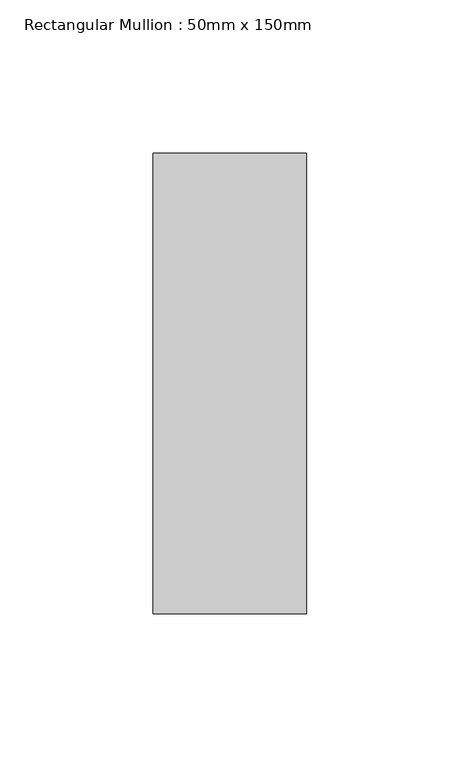
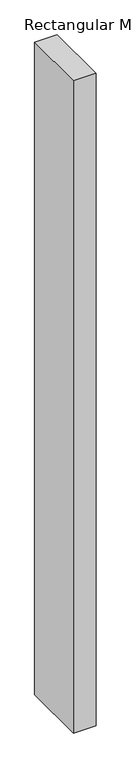
"""IFC4 building model written with IfcOpenShell, lengths in millimetres: member geometry, Rectangular Mullion : 50mm x 150mm."""

from ifc_helpers import new_model, si_unit, frame, origin, place, context, project, spatial, polyline, outline, extrude, source, transform, mapped, element, save


def rectangular_mullion_50mm_x_150mm_b35f0c6e(model_context):
    return source(origin(), model_context, "Body", "SweptSolid", [
        extrude(outline(polyline([(0.0, 75.0), (0.0, -75.0), (-50.0, -75.0), (-50.0, 75.0), (0.0, 75.0)])), frame((0.0, 0.0, -1538.6474098), z_axis=(0.0, 0.0, 1.0), x_axis=(1.0, 0.0, 0.0)), (0.0, 0.0, 1.0), 1538.6474098),
    ])


if __name__ == "__main__":
    model = new_model("IFC4")
    model_context = context("Model", 3, world=origin())
    ifc_project = project(units=[si_unit("LENGTHUNIT", "METRE", prefix="MILLI")], contexts=[model_context])
    site = spatial("IfcSite", under=ifc_project)
    building = spatial("IfcBuilding", under=site)
    placement = place(None, origin())
    rectangular_mullion_50mm_x_150mm_shape = rectangular_mullion_50mm_x_150mm_b35f0c6e(model_context)
    element("IfcMember", 1, ObjectType="Rectangular Mullion : 50mm x 150mm", at=placement, inside=building, context=model_context, shape_type="MappedRepresentation", body=[
        mapped(rectangular_mullion_50mm_x_150mm_shape, transform((0.0, 0.0, 0.0), x_axis=(1.0, 0.0, 0.0), y_axis=(0.0, 1.0, 0.0), z_axis=(0.0, 0.0, 1.0))),
    ])
    save(model, "model.ifc")

# Revit data of these elements
# Type "Rectangular Mullion : 50mm x 150mm"
#   built-in parameter 1007304 = 0.492126 (stored number, unit not read)
#   built-in parameter 1007301 = 0.082021 (stored number, unit not read)
#   built-in parameter 1007300 = 0.082021 (stored number, unit not read)
# Element 1 (IfcMember, "Rectangular Mullion : 50mm x 150mm")
#   Materials on its faces: "Aluminum"
# Materials
#   "Aluminum": class "Metal", colour RGB 244 244 244, transparency 0, Description = "Aluminum 6061", Cost = 0
